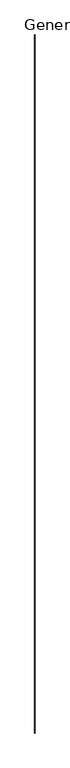
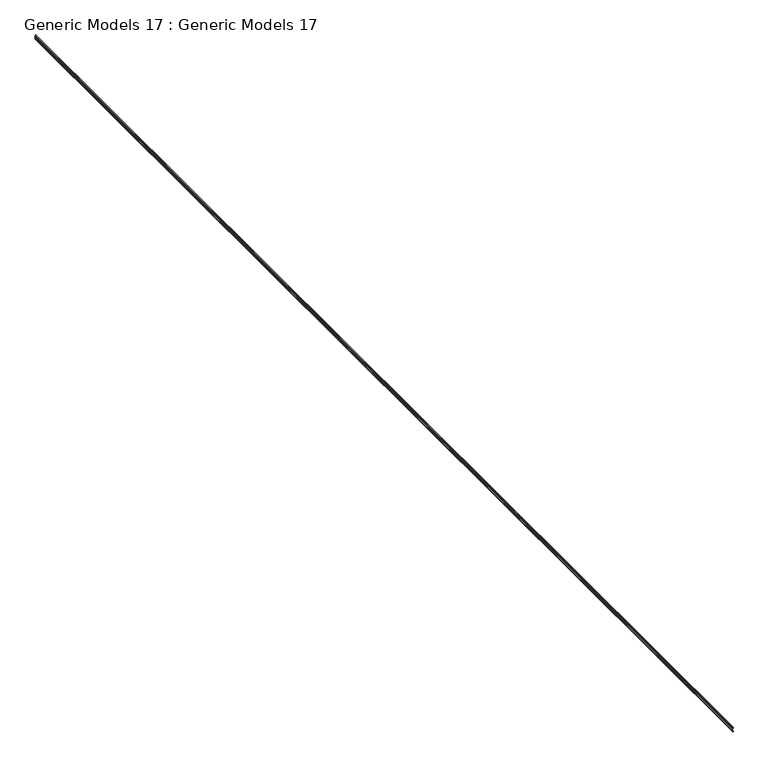
"""IFC4 building model written with IfcOpenShell, lengths in millimetres: proxy geometry, Generic Models 17 : Generic Models 17."""

import ifcopenshell
import ifcopenshell.guid

model = None  # the IFC model being written
_history = None  # IfcOwnerHistory: only IFC2X3 demands one
_inside = {}  # id of a spatial element -> (the spatial element, [elements in it])
_under = {}  # id of a project, library or spatial element -> (it, [spatial elements below it])
_declared = {}  # id of a project -> (the project, [libraries it declares])
_typed = {}  # id of a type object -> (the type object, [elements of that type])
_made_of = {}  # id of a material, layer set ... -> (it, [elements and type objects made of it])


def new_model(schema):
    """Start an empty IFC model of exactly this schema.

    Asked for "IFC4X3", IfcOpenShell would pick the latest addendum, in which some entities
    have other attributes; the version numbers below select the first issue.
    IFC2X3 requires an IfcOwnerHistory on every rooted entity: one is made here for all.
    """
    global model, _history
    if schema == "IFC4X3":
        model = ifcopenshell.file(schema_version=(4, 3, 0, 0))
    else:
        model = ifcopenshell.file(schema=schema)
    _inside.clear()
    _under.clear()
    _declared.clear()
    _typed.clear()
    _made_of.clear()
    _history = None
    if model.schema == "IFC2X3":
        org = make("IfcOrganization", Name="unknown")
        user = make(
            "IfcPersonAndOrganization",
            ThePerson=make("IfcPerson", FamilyName="unknown"),
            TheOrganization=org,
        )
        app = make(
            "IfcApplication",
            ApplicationDeveloper=org,
            Version="unknown",
            ApplicationFullName="unknown",
            ApplicationIdentifier="unknown",
        )
        _history = make(
            "IfcOwnerHistory",
            OwningUser=user,
            OwningApplication=app,
            ChangeAction="ADDED",
            CreationDate=0,
        )
    return model


def make(cls, **values):
    """One entity of the class cls with the attributes given. An attribute that is None is left unset."""
    return model.create_entity(
        cls, **{name: value for name, value in values.items() if value is not None}
    )


def rooted(cls, **values):
    """An entity with a GlobalId (a new one), such as an element, a storey or a relation."""
    return make(cls, GlobalId=ifcopenshell.guid.new(), OwnerHistory=_history, **values)


def si_unit(unit_type, name, prefix=None):
    """IfcSIUnit, for example si_unit("LENGTHUNIT", "METRE", prefix="MILLI")."""
    return make("IfcSIUnit", UnitType=unit_type, Prefix=prefix, Name=name)


def assignment(units):
    """IfcUnitAssignment: the units of a project."""
    return None if units is None else make("IfcUnitAssignment", Units=units)


def point(xyz):
    """IfcCartesianPoint."""
    return None if xyz is None else make("IfcCartesianPoint", Coordinates=xyz)


def direction(xyz):
    """IfcDirection."""
    return None if xyz is None else make("IfcDirection", DirectionRatios=xyz)


def frame(location, z_axis=None, x_axis=None):
    """IfcAxis2Placement3D, a coordinate frame: its origin and axes. An axis left out is left unset."""
    return make(
        "IfcAxis2Placement3D",
        Location=point(location),
        Axis=direction(z_axis),
        RefDirection=direction(x_axis),
    )


def frame_2d(location, x_axis=None):
    """IfcAxis2Placement2D, a coordinate frame in the plane: its origin and x axis."""
    return make(
        "IfcAxis2Placement2D", Location=point(location), RefDirection=direction(x_axis)
    )


def origin():
    """The frame at (0, 0, 0) with its axes left unset."""
    return frame((0.0, 0.0, 0.0))


def place(relative_to, where):
    """IfcLocalPlacement: puts the frame where relative to a parent placement (None: the world)."""
    return make(
        "IfcLocalPlacement", PlacementRelTo=relative_to, RelativePlacement=where
    )


def context(
    kind, dimensions, precision=None, world=None, true_north=None, identifier=None
):
    """IfcGeometricRepresentationContext, for example the 3D "Model" context."""
    return make(
        "IfcGeometricRepresentationContext",
        ContextIdentifier=identifier,
        ContextType=kind,
        CoordinateSpaceDimension=dimensions,
        Precision=precision,
        WorldCoordinateSystem=world,
        TrueNorth=true_north,
    )


def project(units=None, contexts=None):
    """IfcProject with its units and contexts."""
    return rooted(
        "IfcProject",
        Name="project",
        RepresentationContexts=contexts,
        UnitsInContext=assignment(units),
    )


def spatial(cls, under=None, at=None, **own):
    """A site, building, storey or space (cls), placed at a placement, below another one or the project."""
    s = rooted(cls, ObjectPlacement=at, **own)
    if under is not None:
        _under.setdefault(under.id(), (under, []))[1].append(s)
    return s


def polyline(points):
    """IfcPolyline through the points."""
    return make("IfcPolyline", Points=[point(p) for p in points])


def circle_curve(where, radius):
    """IfcCircle in the frame where."""
    return make("IfcCircle", Position=where, Radius=radius)


def trimmed(basis, trim1, trim2, sense, master):
    """IfcTrimmedCurve: the piece of a basis curve between two trims."""
    return make(
        "IfcTrimmedCurve",
        BasisCurve=basis,
        Trim1=trim1,
        Trim2=trim2,
        SenseAgreement=sense,
        MasterRepresentation=master,
    )


def segment(curve, same_sense, transition):
    """IfcCompositeCurveSegment."""
    return make(
        "IfcCompositeCurveSegment",
        Transition=transition,
        SameSense=same_sense,
        ParentCurve=curve,
    )


def composite_curve(segments, self_intersect=None):
    """IfcCompositeCurve: segments joined end to end."""
    return make("IfcCompositeCurve", Segments=segments, SelfIntersect=self_intersect)


def outline(outer, holes=None, kind="AREA"):
    """IfcArbitraryClosedProfileDef: a profile drawn as a closed curve; with holes, ...WithVoids."""
    if holes is None:
        return make("IfcArbitraryClosedProfileDef", ProfileType=kind, OuterCurve=outer)
    return make(
        "IfcArbitraryProfileDefWithVoids",
        ProfileType=kind,
        OuterCurve=outer,
        InnerCurves=holes,
    )


def extrude(swept, where, along, depth):
    """IfcExtrudedAreaSolid: the profile swept, set in the frame where, extruded along a direction by depth."""
    return make(
        "IfcExtrudedAreaSolid",
        SweptArea=swept,
        Position=where,
        ExtrudedDirection=direction(along),
        Depth=depth,
    )


def shape(context_of_items, identifier, shape_type, items):
    """IfcShapeRepresentation: the items that make up one representation, for example the "Body"."""
    return make(
        "IfcShapeRepresentation",
        ContextOfItems=context_of_items,
        RepresentationIdentifier=identifier,
        RepresentationType=shape_type,
        Items=items,
    )


def source(mapping_origin, context_of_items, identifier, shape_type, items):
    """IfcRepresentationMap: a shape defined once, which mapped items show again and again."""
    return make(
        "IfcRepresentationMap",
        MappingOrigin=mapping_origin,
        MappedRepresentation=shape(context_of_items, identifier, shape_type, items),
    )


def transform(
    local_origin,
    x_axis=None,
    y_axis=None,
    z_axis=None,
    scale=None,
    scale2=None,
    scale3=None,
    uniform=True,
):
    """IfcCartesianTransformationOperator3D, or its non-uniform kind. x_axis, y_axis, z_axis: its Axis1, 2, 3."""
    if uniform:
        return make(
            "IfcCartesianTransformationOperator3D",
            Axis1=direction(x_axis),
            Axis2=direction(y_axis),
            LocalOrigin=point(local_origin),
            Scale=scale,
            Axis3=direction(z_axis),
        )
    return make(
        "IfcCartesianTransformationOperator3DnonUniform",
        Axis1=direction(x_axis),
        Axis2=direction(y_axis),
        LocalOrigin=point(local_origin),
        Scale=scale,
        Axis3=direction(z_axis),
        Scale2=scale2,
        Scale3=scale3,
    )


def mapped(mapping_source, mapping_target):
    """IfcMappedItem: shows the shape of a source again, moved by a transform."""
    return make(
        "IfcMappedItem", MappingSource=mapping_source, MappingTarget=mapping_target
    )


def made_of(thing, what):
    """Note that an element or type object is made of a material, layer set ...; save() writes the relation."""
    if what is not None:
        _made_of.setdefault(what.id(), (what, []))[1].append(thing)
    return thing


def element(
    cls,
    number,
    at=None,
    inside=None,
    cuts=None,
    type_object=None,
    material=None,
    context=None,
    identifier="Body",
    shape_type=None,
    held_by="IfcProductDefinitionShape",
    body=None,
    shapes=None,
    **own,
):
    """One element of the class cls, such as IfcWall. Its Tag is "e" and its number.

    at: its placement. inside: the storey or other place that contains it. cuts: it is an
    opening in that element (IfcRelVoidsElement). A single representation is given by context,
    identifier, shape_type and body (its items); several are given by shapes. held_by: the class
    of the entity that holds the representations. save() writes the other relations.
    """
    e = rooted(cls, Tag="e%d" % number, ObjectPlacement=at, **own)
    if body is not None:
        shapes = [shape(context, identifier, shape_type, body)]
    if shapes is not None:
        e.Representation = make(held_by, Representations=shapes)
    if inside is not None:
        _inside.setdefault(inside.id(), (inside, []))[1].append(e)
    if cuts is not None:
        rooted(
            "IfcRelVoidsElement", RelatingBuildingElement=cuts, RelatedOpeningElement=e
        )
    if type_object is not None:
        _typed.setdefault(type_object.id(), (type_object, []))[1].append(e)
    return made_of(e, material)


def aggregate(whole, parts):
    """IfcRelAggregates: a whole, such as a stair, and the parts it consists of."""
    return rooted("IfcRelAggregates", RelatingObject=whole, RelatedObjects=parts)


def save(model, path):
    """Write the relations noted so far, then the file.

    IfcRelAggregates (storeys below a building ...), IfcRelContainedInSpatialStructure (elements
    in a storey), IfcRelDefinesByType, IfcRelAssociatesMaterial and IfcRelDeclares: one each for
    every whole, place, type object, material and project.
    """
    for whole, parts in _under.values():
        aggregate(whole, parts)
    for where, things in _inside.values():
        rooted(
            "IfcRelContainedInSpatialStructure",
            RelatedElements=things,
            RelatingStructure=where,
        )
    for kind, things in _typed.values():
        rooted("IfcRelDefinesByType", RelatedObjects=things, RelatingType=kind)
    for what, things in _made_of.values():
        rooted("IfcRelAssociatesMaterial", RelatedObjects=things, RelatingMaterial=what)
    for by, libraries in _declared.values():
        rooted("IfcRelDeclares", RelatingContext=by, RelatedDefinitions=libraries)
    model.write(path)


def generic_models_17_generic_models_17_78fa32c8(model_context):
    return source(origin(), model_context, "Body", "SweptSolid", [
        extrude(outline(composite_curve([segment(polyline([(271610.6737098, 23402.9215778), (271597.1483788, 23402.9215778), (271597.1483788, 23404.5090778), (271611.9492241, 23404.5090778), (271614.2628473, 23394.0193664)]), True, "CONTINUOUS"), segment(trimmed(circle_curve(frame_2d((271615.0379675, 23394.1903278)), 0.79375), [point((271614.2628473, 23394.0193664))], [point((271615.6295938, 23393.6611611))], True, "CARTESIAN"), True, "CONTINUOUS"), segment(trimmed(circle_curve(frame_2d((271618.5877254, 23391.0153278)), 3.96875), [point((271615.6295938, 23393.6611611))], [point((271618.5877254, 23394.9840778))], False, "CARTESIAN"), True, "CONTINUOUS"), segment(polyline([(271618.5877254, 23394.9840778), (271639.2090323, 23394.9840778)]), True, "CONTINUOUS"), segment(trimmed(circle_curve(frame_2d((271639.2090323, 23391.0153278)), 3.96875), [point((271639.2090323, 23394.9840778))], [point((271642.1671639, 23393.6611611))], False, "CARTESIAN"), True, "CONTINUOUS"), segment(trimmed(circle_curve(frame_2d((271642.7587902, 23394.1903278)), 0.79375), [point((271642.1671639, 23393.6611611))], [point((271643.5339104, 23394.0193664))], True, "CARTESIAN"), True, "CONTINUOUS"), segment(polyline([(271643.5339104, 23394.0193664), (271645.8475336, 23404.5090778), (271660.6483788, 23404.5090778), (271660.6483788, 23402.9215778), (271647.1230479, 23402.9215778), (271645.0841507, 23393.6774436)]), True, "CONTINUOUS"), segment(trimmed(circle_curve(frame_2d((271642.7587902, 23394.1903278)), 2.38125), [point((271645.0841507, 23393.6774436))], [point((271640.9839113, 23392.6028278))], False, "CARTESIAN"), True, "CONTINUOUS"), segment(trimmed(circle_curve(frame_2d((271639.2090323, 23391.0153278)), 2.38125), [point((271640.9839113, 23392.6028278))], [point((271639.2090323, 23393.3965778))], True, "CARTESIAN"), True, "CONTINUOUS"), segment(polyline([(271639.2090323, 23393.3965778), (271618.5877254, 23393.3965778)]), True, "CONTINUOUS"), segment(trimmed(circle_curve(frame_2d((271618.5877254, 23391.0153278)), 2.38125), [point((271618.5877254, 23393.3965778))], [point((271616.8128464, 23392.6028278))], True, "CARTESIAN"), True, "CONTINUOUS"), segment(trimmed(circle_curve(frame_2d((271615.0379675, 23394.1903278)), 2.38125), [point((271616.8128464, 23392.6028278))], [point((271612.712607, 23393.6774436))], False, "CARTESIAN"), True, "CONTINUOUS"), segment(polyline([(271612.712607, 23393.6774436), (271610.6737098, 23402.9215778)]), True, "CONTINUOUS")], self_intersect=False)), frame((0.0, 25500.6656612, 0.0), z_axis=(0.0, 1.0, 0.0), x_axis=(0.0, 0.0, 1.0)), (0.0, 0.0, 1.0), 15480.18875),
    ])


if __name__ == "__main__":
    model = new_model("IFC4")
    model_context = context("Model", 3, world=origin())
    ifc_project = project(units=[si_unit("LENGTHUNIT", "METRE", prefix="MILLI")], contexts=[model_context])
    site = spatial("IfcSite", under=ifc_project)
    building = spatial("IfcBuilding", under=site)
    placement = place(None, origin())
    generic_models_17_generic_models_17_shape = generic_models_17_generic_models_17_78fa32c8(model_context)
    element("IfcBuildingElementProxy", 1, Name="Generic Models 17 : Generic Models 17", ObjectType="Generic Models 17 : Generic Models 17", at=placement, inside=building, context=model_context, shape_type="MappedRepresentation", body=[
        mapped(generic_models_17_generic_models_17_shape, transform((0.0, 0.0, 0.0), x_axis=(1.0, 0.0, 0.0), y_axis=(0.0, 1.0, 0.0), z_axis=(0.0, 0.0, 1.0))),
    ])
    save(model, "model.ifc")

# Revit data of these elements
# Element 1 (IfcBuildingElementProxy, "Generic Models 17 : Generic Models 17")
#   Materials on its faces: "1/2\" DEEP GALV. HORTZ. HAT CHANNEL @ XX O.C."
# Materials
#   "1/2\" DEEP GALV. HORTZ. HAT CHANNEL @ XX O.C.": class "Generic", colour RGB 212 212 212, transparency 0, Cost = 0
